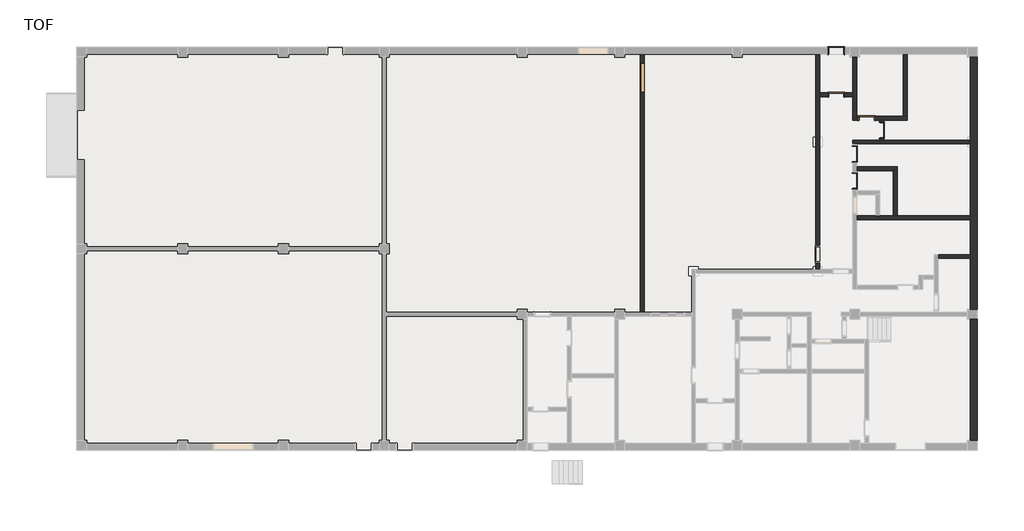
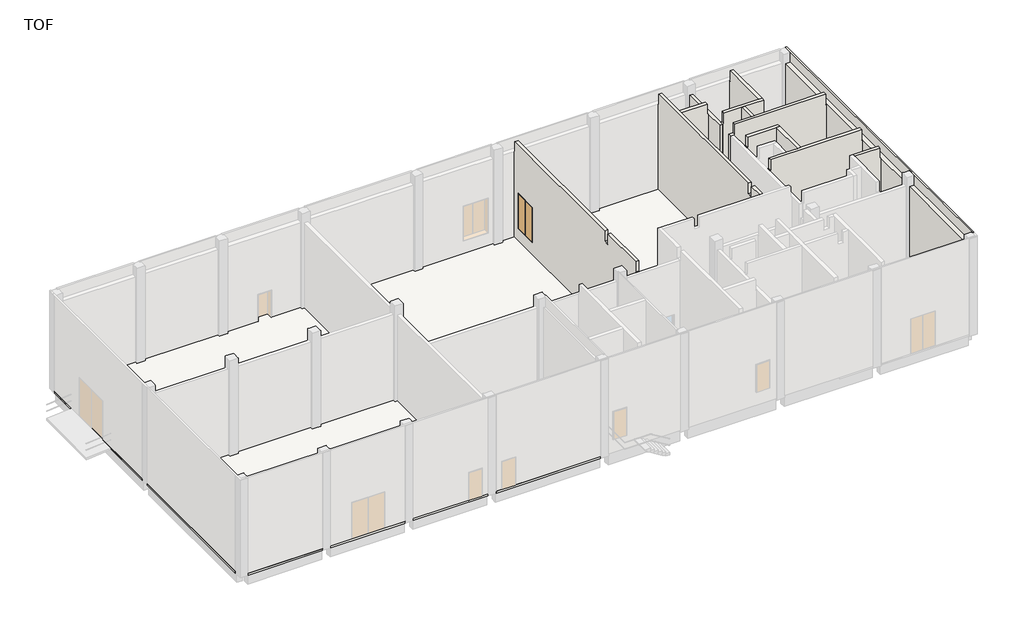
# One storey, part 3 of 5: 13 walls, 7 doors, 2 slabs.
# Revit data of these elements (continued)
# Project information
#   Building Name = "SULFUR LOADING CONTROL BD"
#   Project Status = "Project Status"
#   Client Name = "현대엔지니어링"
#   Project Address = "서울시 종로구 율곡로 75(계동)"
#   Project Number = "-"
# Grids (mm)
#   "Y1": line (-3935.398, 24016.521) -> (58968.688, 24016.521)
#   "X1": line (-75.3, 29394.337) -> (-75.3, -4379.638)
#   "X2": line (5924.7, 29394.337) -> (5924.7, -4379.638)
#   "Y3": line (-3935.398, 8416.521) -> (58968.688, 8416.521)
#   "Y4": line (-3935.398, 616.521) -> (58968.688, 616.521)
#   "X3": line (11924.7, 29394.337) -> (11924.7, -4379.638)
#   "X4": line (17924.7, 29394.337) -> (17924.7, -4379.638)
#   "X5": line (26124.7, 29394.337) -> (26124.7, -4379.638)
#   "X6": line (31924.7, 29394.337) -> (31924.7, -4379.638)
#   "X7": line (38924.7, 29394.337) -> (38924.7, -4379.638)
#   "X8": line (45924.7, 29394.337) -> (45924.7, -4379.638)
#   "X9": line (52924.7, 29394.337) -> (52924.7, -4379.638)
#   "X15": line (43724.7, 27041.858) -> (43724.7, 9156.488)
#   "X16": line (36324.7, 27041.858) -> (36324.7, 9156.488)
#   "X17": line (34685.051, 10966.521) -> (55094.626, 10966.521)
#   "X18": line (34685.051, 18666.521) -> (55094.626, 18666.521)
#   "Y2": line (-3935.398, 12316.521) -> (58968.688, 12316.521)
# Type "Double Door_Steel : H_DR_AMB_Double Door_Steel_W1800xH2700"
#   Type Mark = "363"
#   프레임 = ""
#   철물 = ""
#   유리/마감 = ""
#   위치/개소 = ""
#   부호 = "1/SD"
#   문번호 = ""
#   문기호 = "SD"
#   Analytic Construction = "<None>"
#   Height = 2700.000 mm
#   Width = 1800.000 mm
#   Define Thermal Properties by = 1
#   문 틀 = none
#   문 = none
#   Function = (empty or 0)
#   Assembly Code = ""
#   Wall Closure = (empty or 0)
# Type "Single Door_Steel : H_DR_AMB_Single Door_Steel_W1000xH2150"
#   Type Mark = "364"
#   Analytic Construction = "<None>"
#   프레임 투영 외부. = 25.000 mm
#   프레임 투영 내부. = 25.000 mm
#   프레임 폭 = 75.000 mm
#   Height = 2150.000 mm
#   Width = 1000.000 mm
#   Define Thermal Properties by = 1
#   문 패널 = none
#   문 프레임 = none
#   Function = (empty or 0)
#   Wall Closure = (empty or 0)
# Type "H_FL_AMF_RC Slab_T150"
#   Keynote = ""
#   Type Comments = ""
#   Description = ""
#   Function = 1
#   Layers, outside or top first: 150.000 mm no material (function 1)
# Type "H_WA_AMW_Brick Wall_Ext (0.5B_50_1.0B / Emulsion)"
#   Type Comments = ""
#   Layers, outside or top first: 0.000 mm no material (function 100); 20.000 mm no material (function 2); 115.000 mm no material (function 1); 50.000 mm no material (function 3); 0.000 mm no material (function 100); 230.000 mm no material (function 1); 15.000 mm no material (function 2); 0.000 mm no material (function 100); 0.000 mm no material (function 100)
# Type "H_WA_AMW_Block Wall_Int_T200 (Both Plaster_Emulsion)"
#   Type Comments = ""
#   Layers, outside or top first: 0.000 mm no material (function 100); 12.000 mm no material (function 2); 200.000 mm no material (function 1); 12.000 mm no material (function 2); 10.000 mm no material (function 5)
# Element 1 (IfcDoor, "Double Door_Steel : H_DR_AMB_Double Door_Steel_W1800xH2700")
#   Door Style Name = "Steel Door_Double_Vision_Panic Bar_Transsom"
#   Ref. Door Size = "W2000xH2100 + W2000xH1000"
#   Door Leaf = "Steel"
#   Door Frame = "Steel"
#   Vision = "Vision"
#   Panic = "Panic"
#   Door Style = DDT14
#   Phase Created = New Construction
# Elements 2, 3, 4, 5, 6, 7 (IfcDoor, "Single Door_Steel : H_DR_AMB_Single Door_Steel_W1000xH2150")
#   Door Style Name = "Steel Door_Single"
#   Ref. Door Size = "W1000 x H2100"
#   Door Leaf = "Steel"
#   Door Frame = "Steel"
#   Vision = "N.A"
#   Panic = "N.A"
#   Door Style = SD11
#   Phase Created = New Construction
# Element 8 (IfcSlab, "H_FL_AMF_RC Slab_T150")
#   Height Offset From Level = 50.000 mm
#   Phase Created = New Construction
#   Materials on its faces: "Default Floor"
# Element 9 (IfcSlab, "H_FL_AMF_RC Slab_T150")
#   built-in parameter 1001955 = 1.5708 (stored number, unit not read)
#   Height Offset From Level = 0.000 mm
#   Phase Created = New Construction
#   Materials on its faces: "Default Floor"
# Element 10 (IfcWall, "H_WA_AMW_Brick Wall_Ext (0.5B_50_1.0B / Emulsion)")
#   Mark = "EW4"
#   Wall Loca = "EXT"
#   Wall Style Name = "Concrete Wall+Insulation+Gypsum Board"
#   Wall Base Material-2 = "Glass Wool (Fiberglass)"
#   Wall Base Material-3 = "Concrete Wall"
#   Wall Finish-Ex = "Acrylic Emulsion Paint on Fair Faced Concrete"
#   Top Offset = 0.000 mm
#   Base Offset = 0.000 mm
#   wall height = 7500.000 mm
#   Wall Style No = EW51-1
#   Phase Created = New Construction
#   Base Constraint = TOF
#   Top Constraint = TOC
#   Materials on its faces: "Default Wall"
# Element 11 (IfcWall, "H_WA_AMW_Block Wall_Int_T200 (Both Plaster_Emulsion)")
#   Mark = "W3"
#   Wall Loca = "INT"
#   Wall Style Name = "Block Wall"
#   Wall Ref. = ""
#   Wall Base Material-1 = "Concrete Block"
#   Wall Base Material-2 = ""
#   Wall Base Material-3 = ""
#   Wall Finish-Ex = ""
#   Top Offset = 0.000 mm
#   Base Offset = 0.000 mm
#   wall height = 7500.000 mm
#   Wall Style No = IW21
#   Phase Created = New Construction
#   Base Constraint = TOF
#   Top Constraint = TOC
#   Materials on its faces: "Default Wall"
# Element 12 (IfcWall, "H_WA_AMW_Block Wall_Int_T200 (Both Plaster_Emulsion)")
#   Mark = "W7"
#   Wall Loca = "INT"
#   Wall Style Name = "Block Wall"
#   Wall Ref. = ""
#   Wall Base Material-1 = "Concrete Block"
#   Wall Base Material-2 = ""
#   Wall Base Material-3 = ""
#   Wall Finish-Ex = ""
#   Top Offset = 0.000 mm
#   Base Offset = 0.000 mm
#   wall height = 7500.000 mm
#   Wall Style No = IW21
#   Phase Created = New Construction
#   Base Constraint = TOF
#   Top Constraint = TOC
#   Materials on its faces: "Default Wall"
# Element 13 (IfcWall, "H_WA_AMW_Block Wall_Int_T200 (Both Plaster_Emulsion)")
#   Mark = "W8"
#   Wall Loca = "INT"
#   Wall Style Name = "Block Wall"
#   Wall Ref. = ""
#   Wall Base Material-1 = "Concrete Block"
#   Wall Base Material-2 = ""
#   Wall Base Material-3 = ""
#   Wall Finish-Ex = ""
#   built-in parameter 1001111 = 1000.000 mm
#   Top Offset = 0.000 mm
#   Base Offset = 1000.000 mm
#   wall height = 6500.000 mm
#   Wall Style No = IW21
#   Phase Created = New Construction
#   Base Constraint = TOF
#   Top Constraint = TOC
#   Materials on its faces: "Default Wall"
# Element 14 (IfcWall, "H_WA_AMW_Block Wall_Int_T200 (Both Plaster_Emulsion)")
#   Mark = "W9"
#   Wall Loca = "INT"
#   Wall Style Name = "Block Wall"
#   Wall Ref. = ""
#   Wall Base Material-1 = "Concrete Block"
#   Wall Base Material-2 = ""
#   Wall Base Material-3 = ""
#   Wall Finish-Ex = ""
#   built-in parameter 1001111 = 1000.000 mm
#   Top Offset = 0.000 mm
#   Base Offset = 1000.000 mm
#   wall height = 6500.000 mm
#   Wall Style No = IW21
#   Phase Created = New Construction
#   Base Constraint = TOF
#   Top Constraint = TOC
#   Materials on its faces: "Default Wall"
# Element 15 (IfcWall, "H_WA_AMW_Block Wall_Int_T200 (Both Plaster_Emulsion)")
#   Mark = "W12"
#   Wall Loca = "INT"
#   Wall Style Name = "Block Wall"
#   Wall Ref. = ""
#   Wall Base Material-1 = "Concrete Block"
#   Wall Base Material-2 = ""
#   Wall Base Material-3 = ""
#   Wall Finish-Ex = ""
#   built-in parameter 1001111 = 1000.000 mm
#   Top Offset = 0.000 mm
#   Base Offset = 1000.000 mm
#   wall height = 6500.000 mm
#   Wall Style No = IW21
#   Phase Created = New Construction
#   Base Constraint = TOF
#   Top Constraint = TOC
#   Materials on its faces: "Default Wall"
# Element 16 (IfcWall, "H_WA_AMW_Block Wall_Int_T200 (Both Plaster_Emulsion)")
#   Mark = "W30"
#   Wall Loca = "INT"
#   Wall Style Name = "Block Wall"
#   Wall Ref. = ""
#   Wall Base Material-1 = "Concrete Block"
#   Wall Base Material-2 = ""
#   Wall Base Material-3 = ""
#   Wall Finish-Ex = ""
#   built-in parameter 1001111 = 1000.000 mm
#   Top Offset = 0.000 mm
#   Base Offset = 1000.000 mm
#   wall height = 6500.000 mm
#   Wall Style No = IW21
#   Phase Created = New Construction
#   Base Constraint = TOF
#   Top Constraint = TOC
#   Materials on its faces: "Default Wall"
# Element 17 (IfcWall, "H_WA_AMW_Block Wall_Int_T200 (Both Plaster_Emulsion)")
#   Mark = "W32"
#   Wall Loca = "INT"
#   Wall Style Name = "Block Wall"
#   Wall Ref. = ""
#   Wall Base Material-1 = "Concrete Block"
#   Wall Base Material-2 = ""
#   Wall Base Material-3 = ""
#   Wall Finish-Ex = ""
#   built-in parameter 1001111 = 1000.000 mm
#   Top Offset = 0.000 mm
#   Base Offset = 1000.000 mm
#   wall height = 6500.000 mm
#   Wall Style No = IW21
#   Phase Created = New Construction
#   Base Constraint = TOF
#   Top Constraint = TOC
#   Materials on its faces: "Default Wall"
# Element 18 (IfcWall, "H_WA_AMW_Block Wall_Int_T200 (Both Plaster_Emulsion)")
#   Mark = "W33"
#   Wall Loca = "INT"
#   Wall Style Name = "Block Wall"
#   Wall Ref. = ""
#   Wall Base Material-1 = "Concrete Block"
#   Wall Base Material-2 = ""
#   Wall Base Material-3 = ""
#   Wall Finish-Ex = ""
#   built-in parameter 1001111 = 1000.000 mm
#   Top Offset = 0.000 mm
#   Base Offset = 1000.000 mm
#   wall height = 6500.000 mm
#   Wall Style No = IW21
#   Phase Created = New Construction
#   Base Constraint = TOF
#   Top Constraint = TOC
#   Materials on its faces: "Default Wall"
# Element 19 (IfcWall, "H_WA_AMW_Block Wall_Int_T200 (Both Plaster_Emulsion)")
#   Mark = "W35"
#   Wall Loca = "INT"
#   Wall Style Name = "Block Wall"
#   Wall Ref. = ""
#   Wall Base Material-1 = "Concrete Block"
#   Wall Base Material-2 = ""
#   Wall Base Material-3 = ""
#   Wall Finish-Ex = ""
#   built-in parameter 1001111 = 1000.000 mm
#   Top Offset = 0.000 mm
#   Base Offset = 1000.000 mm
#   wall height = 6500.000 mm
#   Wall Style No = IW21
#   Phase Created = New Construction
#   Base Constraint = TOF
#   Top Constraint = TOC
#   Materials on its faces: "Default Wall"
# Element 20 (IfcWall, "H_WA_AMW_Block Wall_Int_T200 (Both Plaster_Emulsion)")
#   Mark = "W36"
#   Wall Loca = "INT"
#   Wall Style Name = "Block Wall"
#   Wall Ref. = ""
#   Wall Base Material-1 = "Concrete Block"
#   Wall Base Material-2 = ""
#   Wall Base Material-3 = ""
#   Wall Finish-Ex = ""
#   built-in parameter 1001111 = 1000.000 mm
#   Top Offset = 0.000 mm
#   Base Offset = 1000.000 mm
#   wall height = 6500.000 mm
#   Wall Style No = IW21
#   Phase Created = New Construction
#   Base Constraint = TOF
#   Top Constraint = TOC
#   Materials on its faces: "Default Wall"
# Element 21 (IfcWall, "H_WA_AMW_Block Wall_Int_T200 (Both Plaster_Emulsion)")
#   Mark = "W37"
#   Wall Loca = "INT"
#   Wall Style Name = "Block Wall"
#   Wall Ref. = ""
#   Wall Base Material-1 = "Concrete Block"
#   Wall Base Material-2 = ""
#   Wall Base Material-3 = ""
#   Wall Finish-Ex = ""
#   built-in parameter 1001111 = 1000.000 mm
#   Top Offset = 0.000 mm
#   Base Offset = 1000.000 mm
#   wall height = 6500.000 mm
#   Wall Style No = IW21
#   Phase Created = New Construction
#   Base Constraint = TOF
#   Top Constraint = TOC
#   Materials on its faces: "Default Wall"
# Element 22 (IfcWall, "H_WA_AMW_Block Wall_Int_T200 (Both Plaster_Emulsion)")
#   Mark = "W38"
#   Wall Loca = "INT"
#   Wall Style Name = "Block Wall"
#   Wall Ref. = ""
#   Wall Base Material-1 = "Concrete Block"
#   Wall Base Material-2 = ""
#   Wall Base Material-3 = ""
#   Wall Finish-Ex = ""
#   built-in parameter 1001111 = 1000.000 mm
#   Top Offset = 0.000 mm
#   Base Offset = 1000.000 mm
#   wall height = 6500.000 mm
#   Wall Style No = IW21
#   Phase Created = New Construction
#   Base Constraint = TOF
#   Top Constraint = TOC
#   Materials on its faces: "Default Wall"
# Materials
#   "Default Floor": class "Miscellaneous", colour RGB 80 80 80, transparency 0
#   "Default Wall": class "Miscellaneous", colour RGB 80 80 80, transparency 0
